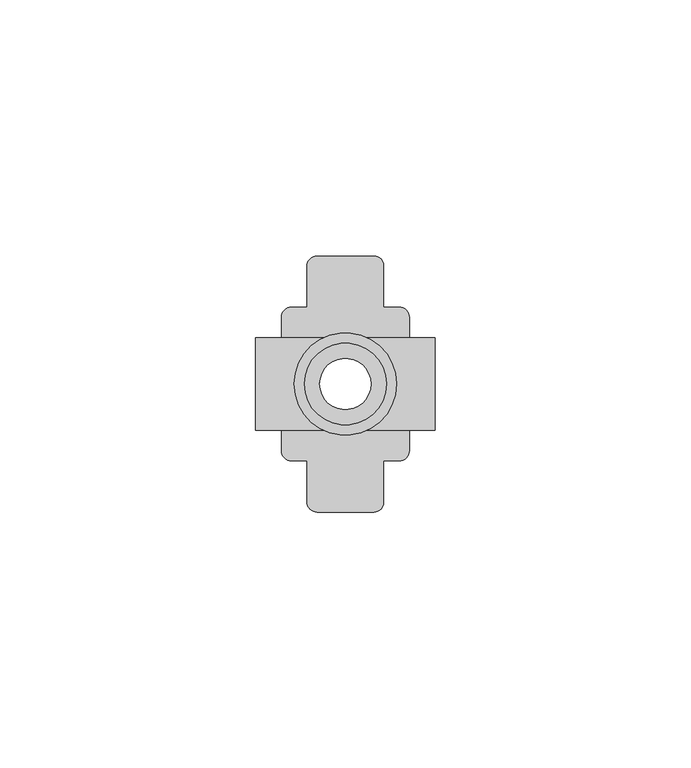
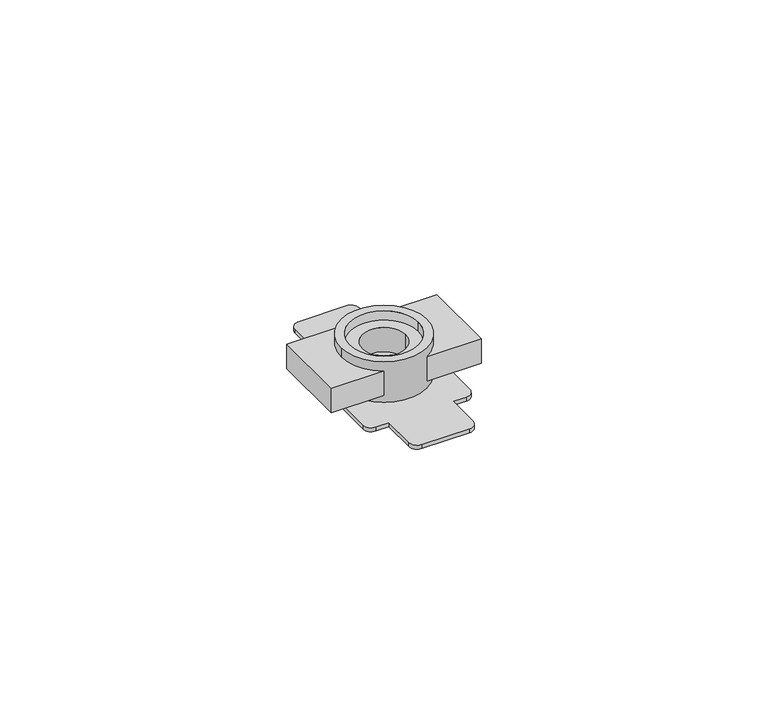
"""IFC4 building model written with IfcOpenShell, lengths in millimetres: proxy geometry, TN_Гайка быстрого монтажа потайная  : Гайка быстрого монтажа потайная 41 8F M10."""

from ifc_helpers import new_model, si_unit, point, frame, frame_2d, origin, origin_2d, place, context, project, spatial, polyline, circle_curve, trimmed, segment, composite_curve, outline, extrude, source, transform, mapped, element, save


def generic_models_8fd2ae9c(model_context):
    return source(origin(), model_context, "Body", "SweptSolid", [
        extrude(outline(composite_curve([segment(trimmed(circle_curve(frame_2d((-10.5188504, 13.0188504)), 1.9811496), [point((-12.5, 13.0188504))], [point((-10.5188504, 15.0))], False, "CARTESIAN"), True, "CONTINUOUS"), segment(polyline([(-10.5188504, 15.0), (-7.5, 15.0), (-7.5, 23.0)]), True, "CONTINUOUS"), segment(trimmed(circle_curve(frame_2d((-5.5, 23.0)), 2.0), [point((-7.5, 23.0))], [point((-5.5, 25.0))], False, "CARTESIAN"), True, "CONTINUOUS"), segment(polyline([(-5.5, 25.0), (5.5634262, 25.0)]), True, "CONTINUOUS"), segment(trimmed(circle_curve(frame_2d((5.5634262, 23.0634262)), 1.9365738), [point((5.5634262, 25.0))], [point((7.5, 23.0634262))], False, "CARTESIAN"), True, "CONTINUOUS"), segment(polyline([(7.5, 23.0634262), (7.5, 15.0), (10.5188504, 15.0)]), True, "CONTINUOUS"), segment(trimmed(circle_curve(frame_2d((10.5188504, 13.0188504)), 1.9811496), [point((10.5188504, 15.0))], [point((12.5, 13.0188504))], False, "CARTESIAN"), True, "CONTINUOUS"), segment(polyline([(12.5, 13.0188504), (12.5, -13.0188504)]), True, "CONTINUOUS"), segment(trimmed(circle_curve(frame_2d((10.5188504, -13.0188504)), 1.9811496), [point((12.5, -13.0188504))], [point((10.5188504, -15.0))], False, "CARTESIAN"), True, "CONTINUOUS"), segment(polyline([(10.5188504, -15.0), (7.5, -15.0), (7.5, -23.0634262)]), True, "CONTINUOUS"), segment(trimmed(circle_curve(frame_2d((5.5634262, -23.0634262)), 1.9365738), [point((7.5, -23.0634262))], [point((5.5634262, -25.0))], False, "CARTESIAN"), True, "CONTINUOUS"), segment(polyline([(5.5634262, -25.0), (-5.5, -25.0)]), True, "CONTINUOUS"), segment(trimmed(circle_curve(frame_2d((-5.5, -23.0)), 2.0), [point((-5.5, -25.0))], [point((-7.5, -23.0))], False, "CARTESIAN"), True, "CONTINUOUS"), segment(polyline([(-7.5, -23.0), (-7.5, -15.0), (-10.5188504, -15.0)]), True, "CONTINUOUS"), segment(trimmed(circle_curve(frame_2d((-10.5188504, -13.0188504)), 1.9811496), [point((-10.5188504, -15.0))], [point((-12.5, -13.0188504))], False, "CARTESIAN"), True, "CONTINUOUS"), segment(polyline([(-12.5, -13.0188504), (-12.5, 13.0188504)]), True, "CONTINUOUS")], self_intersect=False), holes=[composite_curve([segment(trimmed(circle_curve(origin_2d(), 5.0), [point((-5.0, 0.0))], [point((5.0, 0.0))], True, "CARTESIAN"), True, "CONTINUOUS"), segment(trimmed(circle_curve(origin_2d(), 5.0), [point((5.0, 0.0))], [point((-5.0, 0.0))], True, "CARTESIAN"), True, "CONTINUOUS")], self_intersect=False)]), frame((0.0, 0.0, -9.2966688), z_axis=(0.0, 0.0, 1.0), x_axis=(1.0, 0.0, 0.0)), (0.0, 0.0, 1.0), 1.0),
        extrude(outline(composite_curve([segment(trimmed(circle_curve(origin_2d(), 10.0), [point((-10.0, 0.0))], [point((10.0, 0.0))], False, "CARTESIAN"), True, "CONTINUOUS"), segment(trimmed(circle_curve(origin_2d(), 10.0), [point((10.0, 0.0))], [point((-10.0, 0.0))], False, "CARTESIAN"), True, "CONTINUOUS")], self_intersect=False), holes=[composite_curve([segment(trimmed(circle_curve(origin_2d(), 8.0), [point((-8.0, 0.0))], [point((8.0, 0.0))], True, "CARTESIAN"), True, "CONTINUOUS"), segment(trimmed(circle_curve(origin_2d(), 8.0), [point((8.0, 0.0))], [point((-8.0, 0.0))], True, "CARTESIAN"), True, "CONTINUOUS")], self_intersect=False)]), frame((0.0, 0.0, -8.2966688), z_axis=(0.0, 0.0, 1.0), x_axis=(1.0, 0.0, 0.0)), (0.0, 0.0, 1.0), 10.2966688),
        extrude(outline(polyline([(17.5, -9.0), (-17.5, -9.0), (-17.5, 9.0), (17.5, 9.0), (17.5, -9.0)]), holes=[composite_curve([segment(trimmed(circle_curve(origin_2d(), 5.0), [point((-5.0, 0.0))], [point((5.0, 0.0))], True, "CARTESIAN"), True, "CONTINUOUS"), segment(trimmed(circle_curve(origin_2d(), 5.0), [point((5.0, 0.0))], [point((-5.0, 0.0))], True, "CARTESIAN"), True, "CONTINUOUS")], self_intersect=False)]), frame((0.0, 0.0, -6.0), z_axis=(0.0, 0.0, 1.0), x_axis=(1.0, 0.0, 0.0)), (0.0, 0.0, 1.0), 6.0),
    ])


if __name__ == "__main__":
    model = new_model("IFC4")
    model_context = context("Model", 3, world=origin())
    ifc_project = project(units=[si_unit("LENGTHUNIT", "METRE", prefix="MILLI")], contexts=[model_context])
    site = spatial("IfcSite", under=ifc_project)
    building = spatial("IfcBuilding", under=site)
    placement = place(None, origin())
    generic_models_shape = generic_models_8fd2ae9c(model_context)
    element("IfcBuildingElementProxy", 1, Name="TN_Гайка быстрого монтажа потайная  : Гайка быстрого монтажа потайная 41 8F M10", ObjectType="TN_Гайка быстрого монтажа потайная  : Гайка быстрого монтажа потайная 41 8F M10", at=placement, inside=building, context=model_context, shape_type="MappedRepresentation", body=[
        mapped(generic_models_shape, transform((0.0, 0.0, 0.0), x_axis=(1.0, 0.0, 0.0), y_axis=(0.0, 1.0, 0.0), z_axis=(0.0, 0.0, 1.0))),
    ])
    save(model, "model.ifc")

# Revit data of these elements
# Type "TN_Гайка быстрого монтажа потайная  : Гайка быстрого монтажа потайная 41 8F M10"
#   Description = "Для надежного и быстрого закрепления заподлицо монтажных деталей, например, монтажных уголков в канавке тяжелого профиля. Сталь 6 / 8 мм; гальваническое покрытие цинком; полиамид."
#   Manufacturer = "ТехноНИКОЛЬ"
#   Model = "Комплектующие к опорам"
#   URL = "https://nav.tn.ru/knowledge-base/polimernye-membrany/opory-pod-oborudovanie-na-ploskoy-krovle/?sphrase_id=266812"
#   ADSK_Обозначение = "ТехноНИКОЛЬ"
#   ADSK_Наименование краткое = "41 8F M10"
#   ADSK_Наименование = "Гайка быстрого монтажа потайная 41 8F M10"
#   ADSK_Масса_Текст = ""
#   ADSK_Марка = "41 8F M10"
#   ADSK_Код изделия = "660823"
#   ADSK_Завод-изготовитель = "ТехноНИКОЛЬ"
#   ADSK_Единица измерения = "шт."
#   ADSK_Группирование = "Комплектующие к опорам"
#   ADSK_URL страницы изделия = "https://nav.tn.ru/knowledge-base/polimernye-membrany/opory-pod-oborudovanie-na-ploskoy-krovle/?sphrase_id=266812"
#   ADSK_URL документации изделия = ""
#   ADSK_Количество = 1
#   Метриал_Пластик = TN_Пластик_Красный
#   ADSK_Материал = TN_СтальГальванизированная_Серый
#   Default Elevation = 0
# Element 1 (IfcBuildingElementProxy, "TN_Гайка быстрого монтажа потайная  : Гайка быстрого монтажа потайная 41 8F M10")
#   Materials on its faces: "TN_Пластик_Красный", "TN_СтальГальванизированная_Серый"
# Materials
#   "TN_Пластик_Красный": class "Типовые", colour RGB 200 10 50, transparency 0, Cost = 0
#   "TN_СтальГальванизированная_Серый": class "Типовые", colour RGB 206 210 213, transparency 0, Cost = 0
